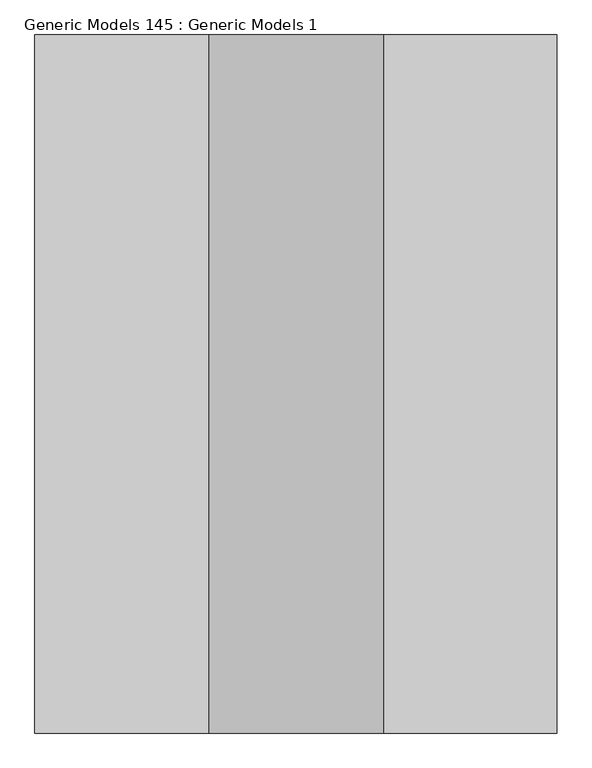
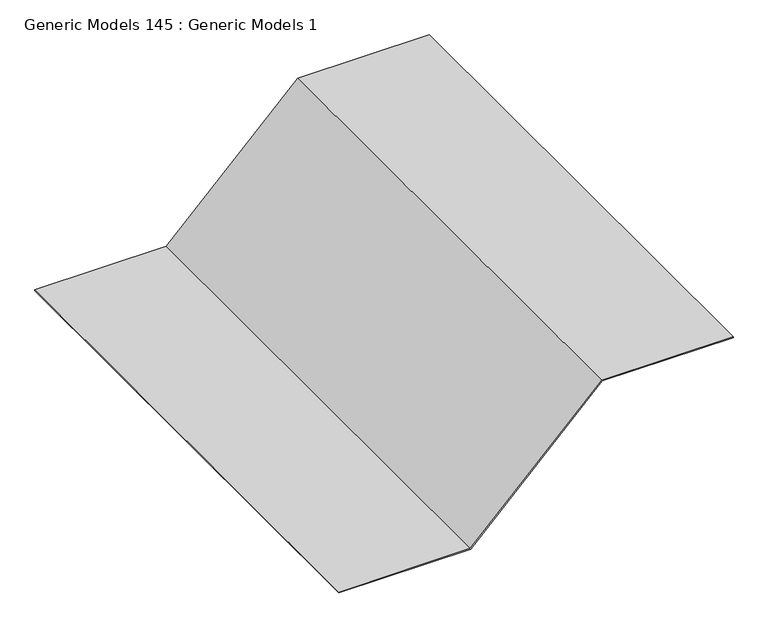
"""IFC4 building model written with IfcOpenShell, lengths in millimetres: proxy geometry, Generic Models 145 : Generic Models 1."""

import ifcopenshell
import ifcopenshell.guid

model = None  # the IFC model being written
_history = None  # IfcOwnerHistory: only IFC2X3 demands one
_inside = {}  # id of a spatial element -> (the spatial element, [elements in it])
_under = {}  # id of a project, library or spatial element -> (it, [spatial elements below it])
_declared = {}  # id of a project -> (the project, [libraries it declares])
_typed = {}  # id of a type object -> (the type object, [elements of that type])
_made_of = {}  # id of a material, layer set ... -> (it, [elements and type objects made of it])


def new_model(schema):
    """Start an empty IFC model of exactly this schema.

    Asked for "IFC4X3", IfcOpenShell would pick the latest addendum, in which some entities
    have other attributes; the version numbers below select the first issue.
    IFC2X3 requires an IfcOwnerHistory on every rooted entity: one is made here for all.
    """
    global model, _history
    if schema == "IFC4X3":
        model = ifcopenshell.file(schema_version=(4, 3, 0, 0))
    else:
        model = ifcopenshell.file(schema=schema)
    _inside.clear()
    _under.clear()
    _declared.clear()
    _typed.clear()
    _made_of.clear()
    _history = None
    if model.schema == "IFC2X3":
        org = make("IfcOrganization", Name="unknown")
        user = make(
            "IfcPersonAndOrganization",
            ThePerson=make("IfcPerson", FamilyName="unknown"),
            TheOrganization=org,
        )
        app = make(
            "IfcApplication",
            ApplicationDeveloper=org,
            Version="unknown",
            ApplicationFullName="unknown",
            ApplicationIdentifier="unknown",
        )
        _history = make(
            "IfcOwnerHistory",
            OwningUser=user,
            OwningApplication=app,
            ChangeAction="ADDED",
            CreationDate=0,
        )
    return model


def make(cls, **values):
    """One entity of the class cls with the attributes given. An attribute that is None is left unset."""
    return model.create_entity(
        cls, **{name: value for name, value in values.items() if value is not None}
    )


def rooted(cls, **values):
    """An entity with a GlobalId (a new one), such as an element, a storey or a relation."""
    return make(cls, GlobalId=ifcopenshell.guid.new(), OwnerHistory=_history, **values)


def si_unit(unit_type, name, prefix=None):
    """IfcSIUnit, for example si_unit("LENGTHUNIT", "METRE", prefix="MILLI")."""
    return make("IfcSIUnit", UnitType=unit_type, Prefix=prefix, Name=name)


def assignment(units):
    """IfcUnitAssignment: the units of a project."""
    return None if units is None else make("IfcUnitAssignment", Units=units)


def point(xyz):
    """IfcCartesianPoint."""
    return None if xyz is None else make("IfcCartesianPoint", Coordinates=xyz)


def direction(xyz):
    """IfcDirection."""
    return None if xyz is None else make("IfcDirection", DirectionRatios=xyz)


def frame(location, z_axis=None, x_axis=None):
    """IfcAxis2Placement3D, a coordinate frame: its origin and axes. An axis left out is left unset."""
    return make(
        "IfcAxis2Placement3D",
        Location=point(location),
        Axis=direction(z_axis),
        RefDirection=direction(x_axis),
    )


def origin():
    """The frame at (0, 0, 0) with its axes left unset."""
    return frame((0.0, 0.0, 0.0))


def place(relative_to, where):
    """IfcLocalPlacement: puts the frame where relative to a parent placement (None: the world)."""
    return make(
        "IfcLocalPlacement", PlacementRelTo=relative_to, RelativePlacement=where
    )


def context(
    kind, dimensions, precision=None, world=None, true_north=None, identifier=None
):
    """IfcGeometricRepresentationContext, for example the 3D "Model" context."""
    return make(
        "IfcGeometricRepresentationContext",
        ContextIdentifier=identifier,
        ContextType=kind,
        CoordinateSpaceDimension=dimensions,
        Precision=precision,
        WorldCoordinateSystem=world,
        TrueNorth=true_north,
    )


def project(units=None, contexts=None):
    """IfcProject with its units and contexts."""
    return rooted(
        "IfcProject",
        Name="project",
        RepresentationContexts=contexts,
        UnitsInContext=assignment(units),
    )


def spatial(cls, under=None, at=None, **own):
    """A site, building, storey or space (cls), placed at a placement, below another one or the project."""
    s = rooted(cls, ObjectPlacement=at, **own)
    if under is not None:
        _under.setdefault(under.id(), (under, []))[1].append(s)
    return s


def polyline(points):
    """IfcPolyline through the points."""
    return make("IfcPolyline", Points=[point(p) for p in points])


def outline(outer, holes=None, kind="AREA"):
    """IfcArbitraryClosedProfileDef: a profile drawn as a closed curve; with holes, ...WithVoids."""
    if holes is None:
        return make("IfcArbitraryClosedProfileDef", ProfileType=kind, OuterCurve=outer)
    return make(
        "IfcArbitraryProfileDefWithVoids",
        ProfileType=kind,
        OuterCurve=outer,
        InnerCurves=holes,
    )


def extrude(swept, where, along, depth):
    """IfcExtrudedAreaSolid: the profile swept, set in the frame where, extruded along a direction by depth."""
    return make(
        "IfcExtrudedAreaSolid",
        SweptArea=swept,
        Position=where,
        ExtrudedDirection=direction(along),
        Depth=depth,
    )


def shape(context_of_items, identifier, shape_type, items):
    """IfcShapeRepresentation: the items that make up one representation, for example the "Body"."""
    return make(
        "IfcShapeRepresentation",
        ContextOfItems=context_of_items,
        RepresentationIdentifier=identifier,
        RepresentationType=shape_type,
        Items=items,
    )


def source(mapping_origin, context_of_items, identifier, shape_type, items):
    """IfcRepresentationMap: a shape defined once, which mapped items show again and again."""
    return make(
        "IfcRepresentationMap",
        MappingOrigin=mapping_origin,
        MappedRepresentation=shape(context_of_items, identifier, shape_type, items),
    )


def transform(
    local_origin,
    x_axis=None,
    y_axis=None,
    z_axis=None,
    scale=None,
    scale2=None,
    scale3=None,
    uniform=True,
):
    """IfcCartesianTransformationOperator3D, or its non-uniform kind. x_axis, y_axis, z_axis: its Axis1, 2, 3."""
    if uniform:
        return make(
            "IfcCartesianTransformationOperator3D",
            Axis1=direction(x_axis),
            Axis2=direction(y_axis),
            LocalOrigin=point(local_origin),
            Scale=scale,
            Axis3=direction(z_axis),
        )
    return make(
        "IfcCartesianTransformationOperator3DnonUniform",
        Axis1=direction(x_axis),
        Axis2=direction(y_axis),
        LocalOrigin=point(local_origin),
        Scale=scale,
        Axis3=direction(z_axis),
        Scale2=scale2,
        Scale3=scale3,
    )


def mapped(mapping_source, mapping_target):
    """IfcMappedItem: shows the shape of a source again, moved by a transform."""
    return make(
        "IfcMappedItem", MappingSource=mapping_source, MappingTarget=mapping_target
    )


def made_of(thing, what):
    """Note that an element or type object is made of a material, layer set ...; save() writes the relation."""
    if what is not None:
        _made_of.setdefault(what.id(), (what, []))[1].append(thing)
    return thing


def element(
    cls,
    number,
    at=None,
    inside=None,
    cuts=None,
    type_object=None,
    material=None,
    context=None,
    identifier="Body",
    shape_type=None,
    held_by="IfcProductDefinitionShape",
    body=None,
    shapes=None,
    **own,
):
    """One element of the class cls, such as IfcWall. Its Tag is "e" and its number.

    at: its placement. inside: the storey or other place that contains it. cuts: it is an
    opening in that element (IfcRelVoidsElement). A single representation is given by context,
    identifier, shape_type and body (its items); several are given by shapes. held_by: the class
    of the entity that holds the representations. save() writes the other relations.
    """
    e = rooted(cls, Tag="e%d" % number, ObjectPlacement=at, **own)
    if body is not None:
        shapes = [shape(context, identifier, shape_type, body)]
    if shapes is not None:
        e.Representation = make(held_by, Representations=shapes)
    if inside is not None:
        _inside.setdefault(inside.id(), (inside, []))[1].append(e)
    if cuts is not None:
        rooted(
            "IfcRelVoidsElement", RelatingBuildingElement=cuts, RelatedOpeningElement=e
        )
    if type_object is not None:
        _typed.setdefault(type_object.id(), (type_object, []))[1].append(e)
    return made_of(e, material)


def aggregate(whole, parts):
    """IfcRelAggregates: a whole, such as a stair, and the parts it consists of."""
    return rooted("IfcRelAggregates", RelatingObject=whole, RelatedObjects=parts)


def save(model, path):
    """Write the relations noted so far, then the file.

    IfcRelAggregates (storeys below a building ...), IfcRelContainedInSpatialStructure (elements
    in a storey), IfcRelDefinesByType, IfcRelAssociatesMaterial and IfcRelDeclares: one each for
    every whole, place, type object, material and project.
    """
    for whole, parts in _under.values():
        aggregate(whole, parts)
    for where, things in _inside.values():
        rooted(
            "IfcRelContainedInSpatialStructure",
            RelatedElements=things,
            RelatingStructure=where,
        )
    for kind, things in _typed.values():
        rooted("IfcRelDefinesByType", RelatedObjects=things, RelatingType=kind)
    for what, things in _made_of.values():
        rooted("IfcRelAssociatesMaterial", RelatedObjects=things, RelatingMaterial=what)
    for by, libraries in _declared.values():
        rooted("IfcRelDeclares", RelatingContext=by, RelatedDefinitions=libraries)
    model.write(path)


def generic_models_145_generic_models_1_d1ee8326(model_context):
    return source(origin(), model_context, "Body", "SweptSolid", [
        extrude(outline(polyline([(-155.575, 52785.9625), (-153.9875, 52785.9625), (-153.9875, 52482.353125), (-458.7875, 52177.553125), (-458.7875, 51873.410689), (-460.375, 51873.410689), (-460.375, 52178.210689), (-155.575, 52483.010689), (-155.575, 52785.9625)])), frame((0.0, 0.0, 0.0), z_axis=(0.0, 1.0, 0.0), x_axis=(0.0, 0.0, 1.0)), (0.0, 0.0, 1.0), 1219.2),
    ])


if __name__ == "__main__":
    model = new_model("IFC4")
    model_context = context("Model", 3, world=origin())
    ifc_project = project(units=[si_unit("LENGTHUNIT", "METRE", prefix="MILLI")], contexts=[model_context])
    site = spatial("IfcSite", under=ifc_project)
    building = spatial("IfcBuilding", under=site)
    placement = place(None, origin())
    generic_models_145_generic_models_1_shape = generic_models_145_generic_models_1_d1ee8326(model_context)
    element("IfcBuildingElementProxy", 1, Name="Generic Models 145 : Generic Models 1", ObjectType="Generic Models 145 : Generic Models 1", at=placement, inside=building, context=model_context, shape_type="MappedRepresentation", body=[
        mapped(generic_models_145_generic_models_1_shape, transform((0.0, 0.0, 0.0), x_axis=(1.0, 0.0, 0.0), y_axis=(0.0, 1.0, 0.0), z_axis=(0.0, 0.0, 1.0))),
    ])
    save(model, "model.ifc")

# Revit data of these elements
# Element 1 (IfcBuildingElementProxy, "Generic Models 145 : Generic Models 1")
#   Materials on its faces: "6 MIL VAPOR BARRIER"
# Materials
#   "6 MIL VAPOR BARRIER": class "Generic", colour RGB 66 158 52, transparency 0, Cost = 0
